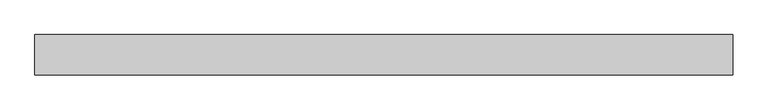
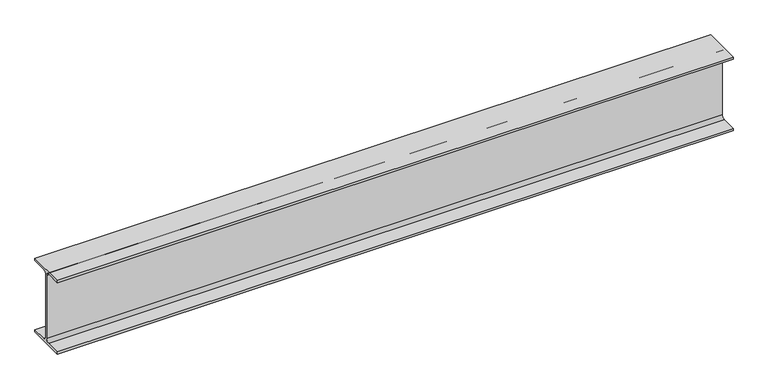
"""IFC4 building model written with IfcOpenShell, lengths in millimetres: beam geometry, Steel Framing_H_KS : H_SB_AR_S02_H-300x150x6.5x9_WG1."""

from ifc_helpers import new_model, si_unit, point, frame, frame_2d, origin, place, context, project, spatial, polyline, circle_curve, trimmed, segment, composite_curve, outline, extrude, source, transform, mapped, element, save


def beam_01aba436(model_context):
    return source(origin(), model_context, "Body", "SweptSolid", [
        extrude(outline(composite_curve([segment(polyline([(75.0, -141.0), (75.0, -150.0), (-75.0, -150.0), (-75.0, -141.0), (-16.25, -141.0)]), True, "CONTINUOUS"), segment(trimmed(circle_curve(frame_2d((-16.25, -128.0)), 13.0), [point((-16.25, -141.0))], [point((-3.25, -128.0))], True, "CARTESIAN"), True, "CONTINUOUS"), segment(polyline([(-3.25, -128.0), (-3.25, 128.0)]), True, "CONTINUOUS"), segment(trimmed(circle_curve(frame_2d((-16.25, 128.0)), 13.0), [point((-3.25, 128.0))], [point((-16.25, 141.0))], True, "CARTESIAN"), True, "CONTINUOUS"), segment(polyline([(-16.25, 141.0), (-75.0, 141.0), (-75.0, 150.0), (75.0, 150.0), (75.0, 141.0), (16.25, 141.0)]), True, "CONTINUOUS"), segment(trimmed(circle_curve(frame_2d((16.25, 128.0)), 13.0), [point((16.25, 141.0))], [point((3.25, 128.0))], True, "CARTESIAN"), True, "CONTINUOUS"), segment(polyline([(3.25, 128.0), (3.25, -128.0)]), True, "CONTINUOUS"), segment(trimmed(circle_curve(frame_2d((16.25, -128.0)), 13.0), [point((3.25, -128.0))], [point((16.25, -141.0))], True, "CARTESIAN"), True, "CONTINUOUS"), segment(polyline([(16.25, -141.0), (75.0, -141.0)]), True, "CONTINUOUS")], self_intersect=False)), frame((-1193.3, 0.0, 0.0), z_axis=(1.0, 0.0, 0.0), x_axis=(0.0, 1.0, 0.0)), (0.0, 0.0, 1.0), 2605.6),
    ])


if __name__ == "__main__":
    model = new_model("IFC4")
    model_context = context("Model", 3, world=origin())
    ifc_project = project(units=[si_unit("LENGTHUNIT", "METRE", prefix="MILLI")], contexts=[model_context])
    site = spatial("IfcSite", under=ifc_project)
    building = spatial("IfcBuilding", under=site)
    placement = place(None, origin())
    beam_shape = beam_01aba436(model_context)
    element("IfcBeam", 1, ObjectType="Steel Framing_H_KS : H_SB_AR_S02_H-300x150x6.5x9_WG1", at=placement, inside=building, context=model_context, shape_type="MappedRepresentation", body=[
        mapped(beam_shape, transform((0.0, 0.0, 0.0), x_axis=(1.0, 0.0, 0.0), y_axis=(0.0, 1.0, 0.0), z_axis=(0.0, 0.0, 1.0))),
    ])
    save(model, "model.ifc")

# Revit data of these elements
# Type "Steel Framing_H_KS : H_SB_AR_S02_H-300x150x6.5x9_WG1"
#   Type Comments = "MAIN"
#   Type Mark = "WG1"
#   H_SectionID = "H-300x150x6.5x9"
#   H_Ratio for Additional Steel Plate = 0.2
#   Width = 15.0 cm
#   Web Thickness = 0.65 cm
#   Web Fillet = 1.3 cm
#   Warping Constant = 107000.0 cm⁶
#   Torsional Moment of Inertia = 9.9539 cm⁴
#   Section Area = 46.78 cm²
#   Plastic Modulus weak axis = 105.0 cm³
#   Plastic Modulus strong axis = 542.0 cm³
#   Perimeter = 1.17 m²/m
#   Nominal Weight = 36.70 kgf/m
#   Moment of Inertia weak axis = 508.00 cm⁴
#   Moment of Inertia strong axis = 7210.00 cm⁴
#   Height = 30.0 cm
#   Flange Thickness = 0.9 cm
#   Elastic Modulus weak axis = 67.7 cm³
#   Elastic Modulus strong axis = 481.0 cm³
#   Centroid Vertical = 15.0 cm
#   Centroid Horizontal = 7.5 cm
#   Bolt Spacing = 8.89 cm
#   Length [instance default] = 1500 mm
#   Structural Material [instance default] = Steel, 45-345
#   Section Name Key = ""
#   Assembly Code = ""
# Element 1 (IfcBeam, "Steel Framing_H_KS : H_SB_AR_S02_H-300x150x6.5x9_WG1")
#   Materials on its faces: "Steel, 45-345"
# Materials
#   "Steel, 45-345": class "Metal", colour RGB 189 187 185, transparency 0, Description = "Steel 345 MPa", Cost = 0
